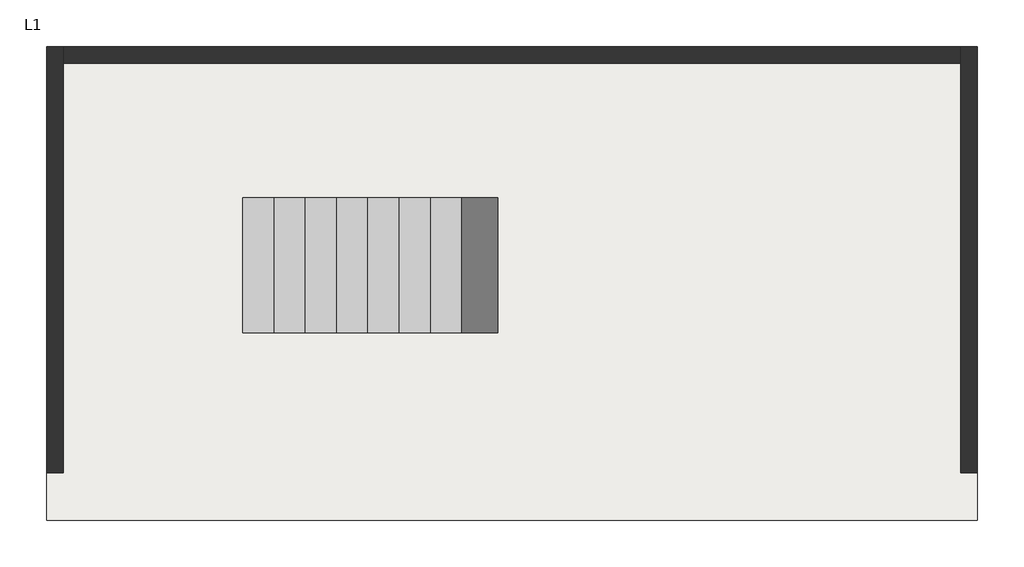
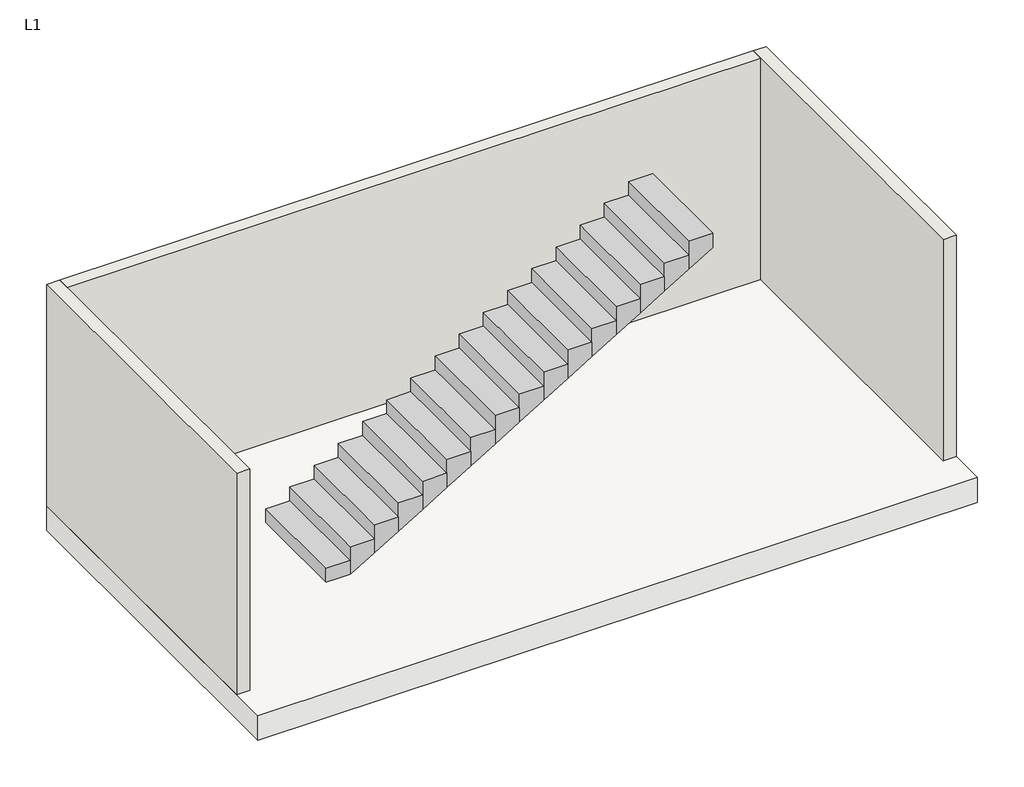
# One storey: 3 walls, 1 slab, 1 stair flight.
"""IFC4 building model written with IfcOpenShell, lengths in millimetres."""

import ifcopenshell
import ifcopenshell.guid

model = None  # the IFC model being written
_history = None  # IfcOwnerHistory: only IFC2X3 demands one
_inside = {}  # id of a spatial element -> (the spatial element, [elements in it])
_under = {}  # id of a project, library or spatial element -> (it, [spatial elements below it])
_declared = {}  # id of a project -> (the project, [libraries it declares])
_typed = {}  # id of a type object -> (the type object, [elements of that type])
_made_of = {}  # id of a material, layer set ... -> (it, [elements and type objects made of it])


def new_model(schema):
    """Start an empty IFC model of exactly this schema.

    Asked for "IFC4X3", IfcOpenShell would pick the latest addendum, in which some entities
    have other attributes; the version numbers below select the first issue.
    IFC2X3 requires an IfcOwnerHistory on every rooted entity: one is made here for all.
    """
    global model, _history
    if schema == "IFC4X3":
        model = ifcopenshell.file(schema_version=(4, 3, 0, 0))
    else:
        model = ifcopenshell.file(schema=schema)
    _inside.clear()
    _under.clear()
    _declared.clear()
    _typed.clear()
    _made_of.clear()
    _history = None
    if model.schema == "IFC2X3":
        org = make("IfcOrganization", Name="unknown")
        user = make(
            "IfcPersonAndOrganization",
            ThePerson=make("IfcPerson", FamilyName="unknown"),
            TheOrganization=org,
        )
        app = make(
            "IfcApplication",
            ApplicationDeveloper=org,
            Version="unknown",
            ApplicationFullName="unknown",
            ApplicationIdentifier="unknown",
        )
        _history = make(
            "IfcOwnerHistory",
            OwningUser=user,
            OwningApplication=app,
            ChangeAction="ADDED",
            CreationDate=0,
        )
    return model


def make(cls, **values):
    """One entity of the class cls with the attributes given. An attribute that is None is left unset."""
    return model.create_entity(
        cls, **{name: value for name, value in values.items() if value is not None}
    )


def rooted(cls, **values):
    """An entity with a GlobalId (a new one), such as an element, a storey or a relation."""
    return make(cls, GlobalId=ifcopenshell.guid.new(), OwnerHistory=_history, **values)


def si_unit(unit_type, name, prefix=None):
    """IfcSIUnit, for example si_unit("LENGTHUNIT", "METRE", prefix="MILLI")."""
    return make("IfcSIUnit", UnitType=unit_type, Prefix=prefix, Name=name)


def assignment(units):
    """IfcUnitAssignment: the units of a project."""
    return None if units is None else make("IfcUnitAssignment", Units=units)


def point(xyz):
    """IfcCartesianPoint."""
    return None if xyz is None else make("IfcCartesianPoint", Coordinates=xyz)


def direction(xyz):
    """IfcDirection."""
    return None if xyz is None else make("IfcDirection", DirectionRatios=xyz)


def frame(location, z_axis=None, x_axis=None):
    """IfcAxis2Placement3D, a coordinate frame: its origin and axes. An axis left out is left unset."""
    return make(
        "IfcAxis2Placement3D",
        Location=point(location),
        Axis=direction(z_axis),
        RefDirection=direction(x_axis),
    )


def origin():
    """The frame at (0, 0, 0) with its axes left unset."""
    return frame((0.0, 0.0, 0.0))


def origin_with_axes():
    """The frame at (0, 0, 0) with the z axis (0, 0, 1) and the x axis (1, 0, 0) written out."""
    return frame((0.0, 0.0, 0.0), z_axis=(0.0, 0.0, 1.0), x_axis=(1.0, 0.0, 0.0))


def place(relative_to, where):
    """IfcLocalPlacement: puts the frame where relative to a parent placement (None: the world)."""
    return make(
        "IfcLocalPlacement", PlacementRelTo=relative_to, RelativePlacement=where
    )


def context(
    kind, dimensions, precision=None, world=None, true_north=None, identifier=None
):
    """IfcGeometricRepresentationContext, for example the 3D "Model" context."""
    return make(
        "IfcGeometricRepresentationContext",
        ContextIdentifier=identifier,
        ContextType=kind,
        CoordinateSpaceDimension=dimensions,
        Precision=precision,
        WorldCoordinateSystem=world,
        TrueNorth=true_north,
    )


def project(units=None, contexts=None):
    """IfcProject with its units and contexts."""
    return rooted(
        "IfcProject",
        Name="project",
        RepresentationContexts=contexts,
        UnitsInContext=assignment(units),
    )


def spatial(cls, under=None, at=None, **own):
    """A site, building, storey or space (cls), placed at a placement, below another one or the project."""
    s = rooted(cls, ObjectPlacement=at, **own)
    if under is not None:
        _under.setdefault(under.id(), (under, []))[1].append(s)
    return s


def polyline(points):
    """IfcPolyline through the points."""
    return make("IfcPolyline", Points=[point(p) for p in points])


def outline(outer, holes=None, kind="AREA"):
    """IfcArbitraryClosedProfileDef: a profile drawn as a closed curve; with holes, ...WithVoids."""
    if holes is None:
        return make("IfcArbitraryClosedProfileDef", ProfileType=kind, OuterCurve=outer)
    return make(
        "IfcArbitraryProfileDefWithVoids",
        ProfileType=kind,
        OuterCurve=outer,
        InnerCurves=holes,
    )


def extrude(swept, where, along, depth):
    """IfcExtrudedAreaSolid: the profile swept, set in the frame where, extruded along a direction by depth."""
    return make(
        "IfcExtrudedAreaSolid",
        SweptArea=swept,
        Position=where,
        ExtrudedDirection=direction(along),
        Depth=depth,
    )


def faces_of(points, faces, orient=None, outer=None):
    """IfcFace entities. A face is a list of loops; a loop is a list of indices into points, from 0.

    orient and outer hold one flag for each loop. By default every Orientation is true, the
    first loop of a face is its IfcFaceOuterBound and the others are IfcFaceBound.
    """
    made = []
    for i, loops in enumerate(faces):
        bounds = []
        for j, loop in enumerate(loops):
            is_outer = j == 0 if outer is None else outer[i][j]
            bounds.append(
                make(
                    "IfcFaceOuterBound" if is_outer else "IfcFaceBound",
                    Bound=make("IfcPolyLoop", Polygon=[points[k] for k in loop]),
                    Orientation=True if orient is None else orient[i][j],
                )
            )
        made.append(make("IfcFace", Bounds=bounds))
    return made


def faceted_brep(points, faces, orient=None, outer=None, voids=None):
    """IfcFacetedBrep: a solid bounded by flat faces; with voids (closed shells), ...WithVoids."""
    shared = [point(p) for p in points]
    hull = make("IfcClosedShell", CfsFaces=faces_of(shared, faces, orient, outer))
    if voids is None:
        return make("IfcFacetedBrep", Outer=hull)
    return make(
        "IfcFacetedBrepWithVoids",
        Outer=hull,
        Voids=[
            make(cls, CfsFaces=faces_of(shared, fs, o, b)) for cls, fs, o, b in voids
        ],
    )


def shape(context_of_items, identifier, shape_type, items):
    """IfcShapeRepresentation: the items that make up one representation, for example the "Body"."""
    return make(
        "IfcShapeRepresentation",
        ContextOfItems=context_of_items,
        RepresentationIdentifier=identifier,
        RepresentationType=shape_type,
        Items=items,
    )


def made_of(thing, what):
    """Note that an element or type object is made of a material, layer set ...; save() writes the relation."""
    if what is not None:
        _made_of.setdefault(what.id(), (what, []))[1].append(thing)
    return thing


def element(
    cls,
    number,
    at=None,
    inside=None,
    cuts=None,
    type_object=None,
    material=None,
    context=None,
    identifier="Body",
    shape_type=None,
    held_by="IfcProductDefinitionShape",
    body=None,
    shapes=None,
    **own,
):
    """One element of the class cls, such as IfcWall. Its Tag is "e" and its number.

    at: its placement. inside: the storey or other place that contains it. cuts: it is an
    opening in that element (IfcRelVoidsElement). A single representation is given by context,
    identifier, shape_type and body (its items); several are given by shapes. held_by: the class
    of the entity that holds the representations. save() writes the other relations.
    """
    e = rooted(cls, Tag="e%d" % number, ObjectPlacement=at, **own)
    if body is not None:
        shapes = [shape(context, identifier, shape_type, body)]
    if shapes is not None:
        e.Representation = make(held_by, Representations=shapes)
    if inside is not None:
        _inside.setdefault(inside.id(), (inside, []))[1].append(e)
    if cuts is not None:
        rooted(
            "IfcRelVoidsElement", RelatingBuildingElement=cuts, RelatedOpeningElement=e
        )
    if type_object is not None:
        _typed.setdefault(type_object.id(), (type_object, []))[1].append(e)
    return made_of(e, material)


def aggregate(whole, parts):
    """IfcRelAggregates: a whole, such as a stair, and the parts it consists of."""
    return rooted("IfcRelAggregates", RelatingObject=whole, RelatedObjects=parts)


def save(model, path):
    """Write the relations noted so far, then the file.

    IfcRelAggregates (storeys below a building ...), IfcRelContainedInSpatialStructure (elements
    in a storey), IfcRelDefinesByType, IfcRelAssociatesMaterial and IfcRelDeclares: one each for
    every whole, place, type object, material and project.
    """
    for whole, parts in _under.values():
        aggregate(whole, parts)
    for where, things in _inside.values():
        rooted(
            "IfcRelContainedInSpatialStructure",
            RelatedElements=things,
            RelatingStructure=where,
        )
    for kind, things in _typed.values():
        rooted("IfcRelDefinesByType", RelatedObjects=things, RelatingType=kind)
    for what, things in _made_of.values():
        rooted("IfcRelAssociatesMaterial", RelatedObjects=things, RelatingMaterial=what)
    for by, libraries in _declared.values():
        rooted("IfcRelDeclares", RelatingContext=by, RelatedDefinitions=libraries)
    model.write(path)


model = new_model("IFC4")

# Units and contexts
model_context = context("Model", 3, world=origin())
ifc_project = project(units=[si_unit("LENGTHUNIT", "METRE", prefix="MILLI")], contexts=[model_context])

# Site, building, storey
site = spatial("IfcSite", under=ifc_project)
building = spatial("IfcBuilding", under=site)
storey = spatial("IfcBuildingStorey", under=building, Name="L1", Elevation=0.0)

# Slab
placement = place(None, origin())
element("IfcSlab", 1, ObjectType="Generic 300mm", at=placement, inside=storey, context=model_context, shape_type="SweptSolid", body=[
    extrude(outline(polyline([(-75.0, 4225.0), (-75.0, 0.0), (-8375.0, 0.0), (-8375.0, 4225.0), (-75.0, 4225.0)])), frame((0.0, 0.0, -300.0), z_axis=(0.0, 0.0, 1.0), x_axis=(1.0, 0.0, 0.0)), (0.0, 0.0, 1.0), 300.0),
])

# Stair flight
element("IfcStairFlight", 2, ObjectType="M_Monolithic Run", at=placement, inside=storey, context=model_context, shape_type="Brep", body=[
    faceted_brep([(-6346.0, 2875.0, 168.75), (-6625.0, 2875.0, 168.75), (-6625.0, 1675.0, 168.75), (-6346.0, 1675.0, 168.75), (-6346.0, 2875.0, 0.0), (-6625.0, 2875.0, 0.0), (-6625.0, 1675.0, 0.0), (-6346.0, 1675.0, 0.0), (-6067.0, 2875.0, 337.5), (-6346.0, 2875.0, 337.5), (-6346.0, 1675.0, 337.5), (-6067.0, 1675.0, 337.5), (-6067.0, 2875.0, 162.196914), (-6335.1655645, 2875.0, 0.0), (-6335.1655645, 1675.0, 0.0), (-6067.0, 1675.0, 162.196914), (-5788.0, 2875.0, 506.25), (-6067.0, 2875.0, 506.25), (-6067.0, 1675.0, 506.25), (-5788.0, 1675.0, 506.25), (-5788.0, 2875.0, 330.946914), (-5788.0, 1675.0, 330.946914), (-5509.0, 2875.0, 675.0), (-5788.0, 2875.0, 675.0), (-5788.0, 1675.0, 675.0), (-5509.0, 1675.0, 675.0), (-5509.0, 2875.0, 499.696914), (-5509.0, 1675.0, 499.696914), (-5230.0, 2875.0, 843.75), (-5509.0, 2875.0, 843.75), (-5509.0, 1675.0, 843.75), (-5230.0, 1675.0, 843.75), (-5230.0, 2875.0, 668.446914), (-5230.0, 1675.0, 668.446914), (-4951.0, 2875.0, 1012.5), (-5230.0, 2875.0, 1012.5), (-5230.0, 1675.0, 1012.5), (-4951.0, 1675.0, 1012.5), (-4951.0, 2875.0, 837.196914), (-4951.0, 1675.0, 837.196914), (-4672.0, 2875.0, 1181.25), (-4951.0, 2875.0, 1181.25), (-4951.0, 1675.0, 1181.25), (-4672.0, 1675.0, 1181.25), (-4672.0, 2875.0, 1005.946914), (-4672.0, 1675.0, 1005.946914), (-4393.0, 2875.0, 1350.0), (-4672.0, 2875.0, 1350.0), (-4672.0, 1675.0, 1350.0), (-4393.0, 1675.0, 1350.0), (-4393.0, 2875.0, 1174.696914), (-4393.0, 1675.0, 1174.696914), (-4114.0, 2875.0, 1518.75), (-4393.0, 2875.0, 1518.75), (-4393.0, 1675.0, 1518.75), (-4114.0, 1675.0, 1518.75), (-4114.0, 2875.0, 1343.446914), (-4114.0, 1675.0, 1343.446914), (-3835.0, 2875.0, 1687.5), (-4114.0, 2875.0, 1687.5), (-4114.0, 1675.0, 1687.5), (-3835.0, 1675.0, 1687.5), (-3835.0, 2875.0, 1512.196914), (-3835.0, 1675.0, 1512.196914), (-3556.0, 2875.0, 1856.25), (-3835.0, 2875.0, 1856.25), (-3835.0, 1675.0, 1856.25), (-3556.0, 1675.0, 1856.25), (-3556.0, 2875.0, 1680.946914), (-3556.0, 1675.0, 1680.946914), (-3277.0, 2875.0, 2025.0), (-3556.0, 2875.0, 2025.0), (-3556.0, 1675.0, 2025.0), (-3277.0, 1675.0, 2025.0), (-3277.0, 2875.0, 1849.696914), (-3277.0, 1675.0, 1849.696914), (-2998.0, 2875.0, 2193.75), (-3277.0, 2875.0, 2193.75), (-3277.0, 1675.0, 2193.75), (-2998.0, 1675.0, 2193.75), (-2998.0, 2875.0, 2018.446914), (-2998.0, 1675.0, 2018.446914), (-2719.0, 2875.0, 2362.5), (-2998.0, 2875.0, 2362.5), (-2998.0, 1675.0, 2362.5), (-2719.0, 1675.0, 2362.5), (-2719.0, 2875.0, 2187.196914), (-2719.0, 1675.0, 2187.196914), (-2440.0, 2875.0, 2531.25), (-2719.0, 2875.0, 2531.25), (-2719.0, 1675.0, 2531.25), (-2440.0, 1675.0, 2531.25), (-2440.0, 2875.0, 2355.946914), (-2440.0, 1675.0, 2355.946914), (-2161.0, 2875.0, 2700.0), (-2440.0, 2875.0, 2700.0), (-2440.0, 1675.0, 2700.0), (-2161.0, 1675.0, 2700.0), (-2161.0, 2875.0, 2524.696914), (-2161.0, 1675.0, 2524.696914)], [[[0, 1, 2, 3]], [[1, 0, 4, 5]], [[2, 1, 5, 6]], [[3, 2, 6, 7]], [[8, 9, 10, 11]], [[4, 0, 9, 8, 12, 13]], [[0, 3, 10, 9]], [[3, 7, 14, 15, 11, 10]], [[16, 17, 18, 19]], [[17, 16, 20, 12, 8]], [[8, 11, 18, 17]], [[19, 18, 11, 15, 21]], [[22, 23, 24, 25]], [[23, 22, 26, 20, 16]], [[16, 19, 24, 23]], [[25, 24, 19, 21, 27]], [[28, 29, 30, 31]], [[29, 28, 32, 26, 22]], [[22, 25, 30, 29]], [[31, 30, 25, 27, 33]], [[34, 35, 36, 37]], [[35, 34, 38, 32, 28]], [[28, 31, 36, 35]], [[37, 36, 31, 33, 39]], [[40, 41, 42, 43]], [[41, 40, 44, 38, 34]], [[34, 37, 42, 41]], [[43, 42, 37, 39, 45]], [[46, 47, 48, 49]], [[47, 46, 50, 44, 40]], [[40, 43, 48, 47]], [[49, 48, 43, 45, 51]], [[52, 53, 54, 55]], [[53, 52, 56, 50, 46]], [[46, 49, 54, 53]], [[55, 54, 49, 51, 57]], [[58, 59, 60, 61]], [[59, 58, 62, 56, 52]], [[52, 55, 60, 59]], [[61, 60, 55, 57, 63]], [[64, 65, 66, 67]], [[65, 64, 68, 62, 58]], [[58, 61, 66, 65]], [[67, 66, 61, 63, 69]], [[70, 71, 72, 73]], [[71, 70, 74, 68, 64]], [[64, 67, 72, 71]], [[73, 72, 67, 69, 75]], [[76, 77, 78, 79]], [[77, 76, 80, 74, 70]], [[70, 73, 78, 77]], [[79, 78, 73, 75, 81]], [[82, 83, 84, 85]], [[83, 82, 86, 80, 76]], [[76, 79, 84, 83]], [[85, 84, 79, 81, 87]], [[88, 89, 90, 91]], [[89, 88, 92, 86, 82]], [[82, 85, 90, 89]], [[91, 90, 85, 87, 93]], [[94, 95, 96, 97]], [[95, 94, 98, 92, 88]], [[88, 91, 96, 95]], [[97, 96, 91, 93, 99]], [[94, 97, 99, 98]], [[5, 4, 13, 14, 7, 6]], [[14, 13, 12, 20, 26, 32, 38, 44, 50, 56, 62, 68, 74, 80, 86, 92, 98, 99, 93, 87, 81, 75, 69, 63, 57, 51, 45, 39, 33, 27, 21, 15]]]),
])

# Walls
element("IfcWall", 3, ObjectType="Generic - 150mm", at=placement, inside=storey, context=model_context, shape_type="Brep", body=[
    faceted_brep([(-75.0, 425.0, 0.0), (-75.0, 4225.0, 0.0), (-75.0, 4225.0, 2700.0), (-75.0, 425.0, 2700.0), (-225.0, 425.0, 0.0), (-225.0, 425.0, 2700.0), (-225.0, 4075.0, 2700.0), (-225.0, 4225.0, 2700.0), (-225.0, 4225.0, 0.0), (-225.0, 4075.0, 0.0)], [[[0, 1, 2, 3]], [[4, 5, 6, 7, 8, 9]], [[1, 0, 4, 9, 8]], [[3, 2, 7, 6, 5]], [[0, 3, 5, 4]], [[2, 1, 8, 7]]]),
])
element("IfcWall", 4, ObjectType="Generic - 150mm", at=placement, inside=storey, context=model_context, shape_type="Brep", body=[
    faceted_brep([(-8375.0, 4225.0, 0.0), (-8375.0, 425.0, 0.0), (-8375.0, 425.0, 2700.0), (-8375.0, 4225.0, 2700.0), (-8225.0, 4225.0, 0.0), (-8225.0, 4225.0, 2700.0), (-8225.0, 4075.0, 2700.0), (-8225.0, 425.0, 2700.0), (-8225.0, 425.0, 0.0), (-8225.0, 4075.0, 0.0)], [[[0, 1, 2, 3]], [[4, 5, 6, 7, 8, 9]], [[1, 0, 4, 9, 8]], [[2, 1, 8, 7]], [[3, 2, 7, 6, 5]], [[0, 3, 5, 4]]]),
])
element("IfcWall", 5, ObjectType="Generic - 150mm", at=placement, inside=storey, context=model_context, shape_type="SweptSolid", body=[
    extrude(outline(polyline([(-225.0, 4075.0), (-8225.0, 4075.0), (-8225.0, 4225.0), (-225.0, 4225.0), (-225.0, 4075.0)])), origin_with_axes(), (0.0, 0.0, 1.0), 2700.0),
])

save(model, "model.ifc")

# Revit data of these elements
# Project information
#   Название организации = "Organization Name"
#   Описание организации = "Organization Description"
#   Наименование здания = "Building Name"
#   Дата утверждения проекта = "Issue Date"
#   Статус проекта = "Project Status"
#   Заказчик = "Client Name"
#   Адрес проекта = "Enter address here\nAddress Line 2"
#   Наименование проекта = "Project Name"
#   Номер проекта = "Project Number"
# Type "Generic 300mm"
#   Description = "Generic Floor (Material By Category), 300mm thick"
#   Function = 0
#   Layers, outside or top first: 300 mm no material (function 1)
# Type "Generic - 150mm"
#   Description = "Generic Wall (Material By Category), 150mm thick"
#   Type Mark = "G04"
#   Layers, outside or top first: 150 mm no material (function 1)
# Element 1 (IfcSlab, "Generic 300mm")
#   Height Offset From Level = 0 mm
#   Phase Created = New Construction
#   Materials on its faces: "Default Floor"
# Element 2 (IfcStairFlight, "M_Monolithic Run")
#   Phase Created = New Construction
# Elements 3, 4, 5 (IfcWall, "Generic - 150mm")
#   Top Offset = 0 mm
#   Base Offset = 0 mm
#   Unconnected Height = 2700 mm
#   wall height = 2700 mm
#   Phase Created = New Construction
#   Base Constraint = L1
#   Materials on its faces: "Default Wall"
# Materials
#   "Default Floor": class "Miscellaneous", colour RGB 128 128 128, transparency 0, Cost = 0
#   "Default Wall": class "Miscellaneous", colour RGB 192 192 192, transparency 0, Cost = 0
